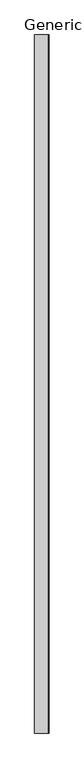
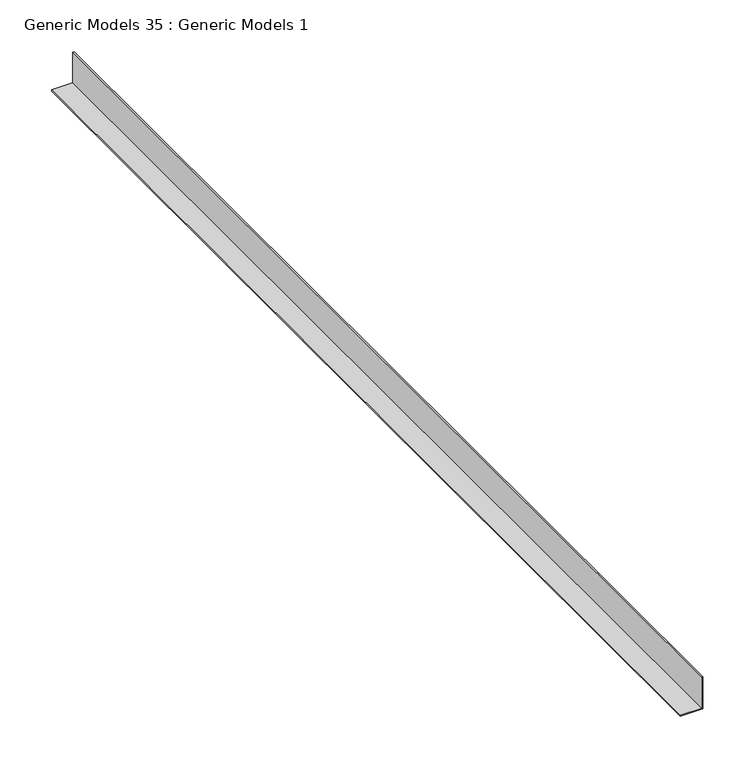
"""IFC4 building model written with IfcOpenShell, lengths in millimetres: proxy geometry, Generic Models 35 : Generic Models 1."""

import ifcopenshell
import ifcopenshell.guid

model = None  # the IFC model being written
_history = None  # IfcOwnerHistory: only IFC2X3 demands one
_inside = {}  # id of a spatial element -> (the spatial element, [elements in it])
_under = {}  # id of a project, library or spatial element -> (it, [spatial elements below it])
_declared = {}  # id of a project -> (the project, [libraries it declares])
_typed = {}  # id of a type object -> (the type object, [elements of that type])
_made_of = {}  # id of a material, layer set ... -> (it, [elements and type objects made of it])


def new_model(schema):
    """Start an empty IFC model of exactly this schema.

    Asked for "IFC4X3", IfcOpenShell would pick the latest addendum, in which some entities
    have other attributes; the version numbers below select the first issue.
    IFC2X3 requires an IfcOwnerHistory on every rooted entity: one is made here for all.
    """
    global model, _history
    if schema == "IFC4X3":
        model = ifcopenshell.file(schema_version=(4, 3, 0, 0))
    else:
        model = ifcopenshell.file(schema=schema)
    _inside.clear()
    _under.clear()
    _declared.clear()
    _typed.clear()
    _made_of.clear()
    _history = None
    if model.schema == "IFC2X3":
        org = make("IfcOrganization", Name="unknown")
        user = make(
            "IfcPersonAndOrganization",
            ThePerson=make("IfcPerson", FamilyName="unknown"),
            TheOrganization=org,
        )
        app = make(
            "IfcApplication",
            ApplicationDeveloper=org,
            Version="unknown",
            ApplicationFullName="unknown",
            ApplicationIdentifier="unknown",
        )
        _history = make(
            "IfcOwnerHistory",
            OwningUser=user,
            OwningApplication=app,
            ChangeAction="ADDED",
            CreationDate=0,
        )
    return model


def make(cls, **values):
    """One entity of the class cls with the attributes given. An attribute that is None is left unset."""
    return model.create_entity(
        cls, **{name: value for name, value in values.items() if value is not None}
    )


def rooted(cls, **values):
    """An entity with a GlobalId (a new one), such as an element, a storey or a relation."""
    return make(cls, GlobalId=ifcopenshell.guid.new(), OwnerHistory=_history, **values)


def si_unit(unit_type, name, prefix=None):
    """IfcSIUnit, for example si_unit("LENGTHUNIT", "METRE", prefix="MILLI")."""
    return make("IfcSIUnit", UnitType=unit_type, Prefix=prefix, Name=name)


def assignment(units):
    """IfcUnitAssignment: the units of a project."""
    return None if units is None else make("IfcUnitAssignment", Units=units)


def point(xyz):
    """IfcCartesianPoint."""
    return None if xyz is None else make("IfcCartesianPoint", Coordinates=xyz)


def direction(xyz):
    """IfcDirection."""
    return None if xyz is None else make("IfcDirection", DirectionRatios=xyz)


def frame(location, z_axis=None, x_axis=None):
    """IfcAxis2Placement3D, a coordinate frame: its origin and axes. An axis left out is left unset."""
    return make(
        "IfcAxis2Placement3D",
        Location=point(location),
        Axis=direction(z_axis),
        RefDirection=direction(x_axis),
    )


def origin():
    """The frame at (0, 0, 0) with its axes left unset."""
    return frame((0.0, 0.0, 0.0))


def place(relative_to, where):
    """IfcLocalPlacement: puts the frame where relative to a parent placement (None: the world)."""
    return make(
        "IfcLocalPlacement", PlacementRelTo=relative_to, RelativePlacement=where
    )


def context(
    kind, dimensions, precision=None, world=None, true_north=None, identifier=None
):
    """IfcGeometricRepresentationContext, for example the 3D "Model" context."""
    return make(
        "IfcGeometricRepresentationContext",
        ContextIdentifier=identifier,
        ContextType=kind,
        CoordinateSpaceDimension=dimensions,
        Precision=precision,
        WorldCoordinateSystem=world,
        TrueNorth=true_north,
    )


def project(units=None, contexts=None):
    """IfcProject with its units and contexts."""
    return rooted(
        "IfcProject",
        Name="project",
        RepresentationContexts=contexts,
        UnitsInContext=assignment(units),
    )


def spatial(cls, under=None, at=None, **own):
    """A site, building, storey or space (cls), placed at a placement, below another one or the project."""
    s = rooted(cls, ObjectPlacement=at, **own)
    if under is not None:
        _under.setdefault(under.id(), (under, []))[1].append(s)
    return s


def polyline(points):
    """IfcPolyline through the points."""
    return make("IfcPolyline", Points=[point(p) for p in points])


def outline(outer, holes=None, kind="AREA"):
    """IfcArbitraryClosedProfileDef: a profile drawn as a closed curve; with holes, ...WithVoids."""
    if holes is None:
        return make("IfcArbitraryClosedProfileDef", ProfileType=kind, OuterCurve=outer)
    return make(
        "IfcArbitraryProfileDefWithVoids",
        ProfileType=kind,
        OuterCurve=outer,
        InnerCurves=holes,
    )


def extrude(swept, where, along, depth):
    """IfcExtrudedAreaSolid: the profile swept, set in the frame where, extruded along a direction by depth."""
    return make(
        "IfcExtrudedAreaSolid",
        SweptArea=swept,
        Position=where,
        ExtrudedDirection=direction(along),
        Depth=depth,
    )


def shape(context_of_items, identifier, shape_type, items):
    """IfcShapeRepresentation: the items that make up one representation, for example the "Body"."""
    return make(
        "IfcShapeRepresentation",
        ContextOfItems=context_of_items,
        RepresentationIdentifier=identifier,
        RepresentationType=shape_type,
        Items=items,
    )


def source(mapping_origin, context_of_items, identifier, shape_type, items):
    """IfcRepresentationMap: a shape defined once, which mapped items show again and again."""
    return make(
        "IfcRepresentationMap",
        MappingOrigin=mapping_origin,
        MappedRepresentation=shape(context_of_items, identifier, shape_type, items),
    )


def transform(
    local_origin,
    x_axis=None,
    y_axis=None,
    z_axis=None,
    scale=None,
    scale2=None,
    scale3=None,
    uniform=True,
):
    """IfcCartesianTransformationOperator3D, or its non-uniform kind. x_axis, y_axis, z_axis: its Axis1, 2, 3."""
    if uniform:
        return make(
            "IfcCartesianTransformationOperator3D",
            Axis1=direction(x_axis),
            Axis2=direction(y_axis),
            LocalOrigin=point(local_origin),
            Scale=scale,
            Axis3=direction(z_axis),
        )
    return make(
        "IfcCartesianTransformationOperator3DnonUniform",
        Axis1=direction(x_axis),
        Axis2=direction(y_axis),
        LocalOrigin=point(local_origin),
        Scale=scale,
        Axis3=direction(z_axis),
        Scale2=scale2,
        Scale3=scale3,
    )


def mapped(mapping_source, mapping_target):
    """IfcMappedItem: shows the shape of a source again, moved by a transform."""
    return make(
        "IfcMappedItem", MappingSource=mapping_source, MappingTarget=mapping_target
    )


def made_of(thing, what):
    """Note that an element or type object is made of a material, layer set ...; save() writes the relation."""
    if what is not None:
        _made_of.setdefault(what.id(), (what, []))[1].append(thing)
    return thing


def element(
    cls,
    number,
    at=None,
    inside=None,
    cuts=None,
    type_object=None,
    material=None,
    context=None,
    identifier="Body",
    shape_type=None,
    held_by="IfcProductDefinitionShape",
    body=None,
    shapes=None,
    **own,
):
    """One element of the class cls, such as IfcWall. Its Tag is "e" and its number.

    at: its placement. inside: the storey or other place that contains it. cuts: it is an
    opening in that element (IfcRelVoidsElement). A single representation is given by context,
    identifier, shape_type and body (its items); several are given by shapes. held_by: the class
    of the entity that holds the representations. save() writes the other relations.
    """
    e = rooted(cls, Tag="e%d" % number, ObjectPlacement=at, **own)
    if body is not None:
        shapes = [shape(context, identifier, shape_type, body)]
    if shapes is not None:
        e.Representation = make(held_by, Representations=shapes)
    if inside is not None:
        _inside.setdefault(inside.id(), (inside, []))[1].append(e)
    if cuts is not None:
        rooted(
            "IfcRelVoidsElement", RelatingBuildingElement=cuts, RelatedOpeningElement=e
        )
    if type_object is not None:
        _typed.setdefault(type_object.id(), (type_object, []))[1].append(e)
    return made_of(e, material)


def aggregate(whole, parts):
    """IfcRelAggregates: a whole, such as a stair, and the parts it consists of."""
    return rooted("IfcRelAggregates", RelatingObject=whole, RelatedObjects=parts)


def save(model, path):
    """Write the relations noted so far, then the file.

    IfcRelAggregates (storeys below a building ...), IfcRelContainedInSpatialStructure (elements
    in a storey), IfcRelDefinesByType, IfcRelAssociatesMaterial and IfcRelDeclares: one each for
    every whole, place, type object, material and project.
    """
    for whole, parts in _under.values():
        aggregate(whole, parts)
    for where, things in _inside.values():
        rooted(
            "IfcRelContainedInSpatialStructure",
            RelatedElements=things,
            RelatingStructure=where,
        )
    for kind, things in _typed.values():
        rooted("IfcRelDefinesByType", RelatedObjects=things, RelatingType=kind)
    for what, things in _made_of.values():
        rooted("IfcRelAssociatesMaterial", RelatedObjects=things, RelatingMaterial=what)
    for by, libraries in _declared.values():
        rooted("IfcRelDeclares", RelatingContext=by, RelatedDefinitions=libraries)
    model.write(path)


def generic_models_35_generic_models_1_f99cc74d(model_context):
    return source(origin(), model_context, "Body", "SweptSolid", [
        extrude(outline(polyline([(2277.1204978, 49676.05), (2277.1204978, 49674.4625), (2240.6079978, 49674.4625), (2240.6079978, 49650.65), (2239.0204978, 49650.65), (2239.0204978, 49676.05), (2277.1204978, 49676.05)])), frame((0.0, 0.0, 0.0), z_axis=(0.0, 1.0, 0.0), x_axis=(0.0, 0.0, 1.0)), (0.0, 0.0, 1.0), 1219.2),
    ])


if __name__ == "__main__":
    model = new_model("IFC4")
    model_context = context("Model", 3, world=origin())
    ifc_project = project(units=[si_unit("LENGTHUNIT", "METRE", prefix="MILLI")], contexts=[model_context])
    site = spatial("IfcSite", under=ifc_project)
    building = spatial("IfcBuilding", under=site)
    placement = place(None, origin())
    generic_models_35_generic_models_1_shape = generic_models_35_generic_models_1_f99cc74d(model_context)
    element("IfcBuildingElementProxy", 1, Name="Generic Models 35 : Generic Models 1", ObjectType="Generic Models 35 : Generic Models 1", at=placement, inside=building, context=model_context, shape_type="MappedRepresentation", body=[
        mapped(generic_models_35_generic_models_1_shape, transform((0.0, 0.0, 0.0), x_axis=(1.0, 0.0, 0.0), y_axis=(0.0, 1.0, 0.0), z_axis=(0.0, 0.0, 1.0))),
    ])
    save(model, "model.ifc")

# Revit data of these elements
# Element 1 (IfcBuildingElementProxy, "Generic Models 35 : Generic Models 1")
#   Materials on its faces: "CEILING TRACK AS SCHEDULED"
# Materials
#   "CEILING TRACK AS SCHEDULED": class "Unassigned", colour RGB 210 209 208, transparency 0, Keynote = "M05121300.02", Cost = 0
